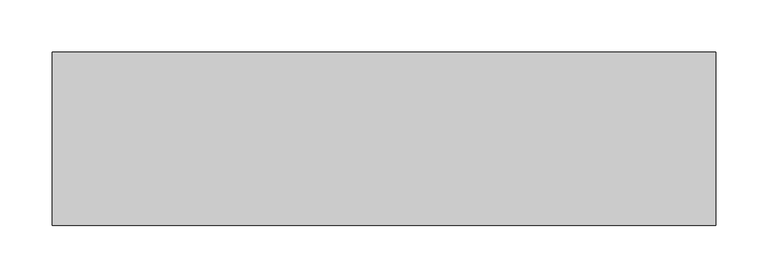
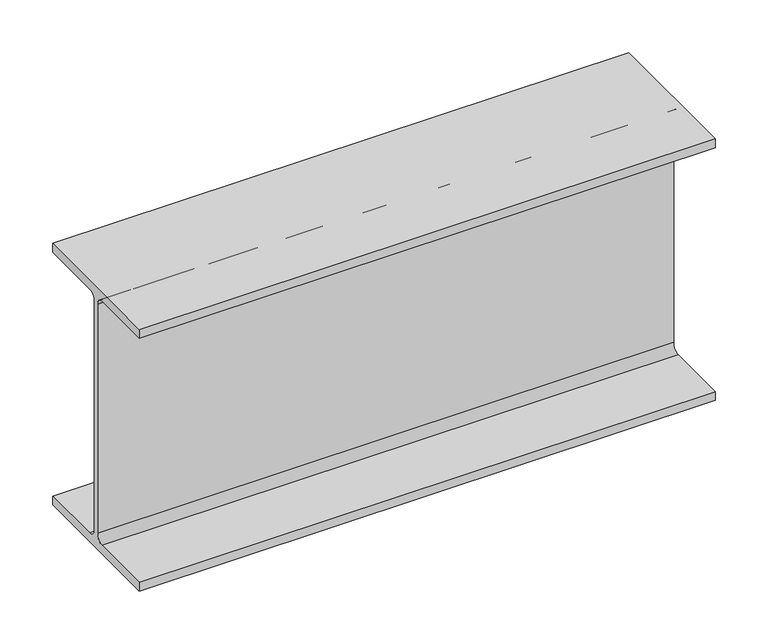
"""IFC4 building model written with IfcOpenShell, lengths in millimetres: beam geometry, Old_Steel Beam_H-KSD3502 : H_SB_ASB_H-300×150x6.5x9."""

from ifc_helpers import new_model, si_unit, point, frame, frame_2d, origin, place, context, project, spatial, polyline, circle_curve, trimmed, segment, composite_curve, outline, extrude, source, transform, mapped, element, save


def beam_aa7ca716(model_context):
    return source(origin(), model_context, "Body", "SweptSolid", [
        extrude(outline(composite_curve([segment(polyline([(-82.5, -141.5), (-11.9, -141.5)]), True, "CONTINUOUS"), segment(trimmed(circle_curve(frame_2d((-11.9, -132.6)), 8.9), [point((-11.9, -141.5))], [point((-3.0, -132.6))], True, "CARTESIAN"), True, "CONTINUOUS"), segment(polyline([(-3.0, -132.6), (-3.0, 132.6)]), True, "CONTINUOUS"), segment(trimmed(circle_curve(frame_2d((-11.9, 132.6)), 8.9), [point((-3.0, 132.6))], [point((-11.9, 141.5))], True, "CARTESIAN"), True, "CONTINUOUS"), segment(polyline([(-11.9, 141.5), (-82.5, 141.5), (-82.5, 151.7), (82.5, 151.7), (82.5, 141.5), (11.9, 141.5)]), True, "CONTINUOUS"), segment(trimmed(circle_curve(frame_2d((11.9, 132.6)), 8.9), [point((11.9, 141.5))], [point((3.0, 132.6))], True, "CARTESIAN"), True, "CONTINUOUS"), segment(polyline([(3.0, 132.6), (3.0, -132.6)]), True, "CONTINUOUS"), segment(trimmed(circle_curve(frame_2d((11.9, -132.6)), 8.9), [point((3.0, -132.6))], [point((11.9, -141.5))], True, "CARTESIAN"), True, "CONTINUOUS"), segment(polyline([(11.9, -141.5), (82.5, -141.5), (82.5, -151.7), (-82.5, -151.7), (-82.5, -141.5)]), True, "CONTINUOUS")], self_intersect=False)), frame((-282.3, 0.0, 0.0), z_axis=(1.0, 0.0, 0.0), x_axis=(0.0, 1.0, 0.0)), (0.0, 0.0, 1.0), 632.1),
    ])


if __name__ == "__main__":
    model = new_model("IFC4")
    model_context = context("Model", 3, world=origin())
    ifc_project = project(units=[si_unit("LENGTHUNIT", "METRE", prefix="MILLI")], contexts=[model_context])
    site = spatial("IfcSite", under=ifc_project)
    building = spatial("IfcBuilding", under=site)
    placement = place(None, origin())
    beam_shape = beam_aa7ca716(model_context)
    element("IfcBeam", 1, ObjectType="Old_Steel Beam_H-KSD3502 : H_SB_ASB_H-300×150x6.5x9", at=placement, inside=building, context=model_context, shape_type="MappedRepresentation", body=[
        mapped(beam_shape, transform((0.0, 0.0, 0.0), x_axis=(1.0, 0.0, 0.0), y_axis=(0.0, 1.0, 0.0), z_axis=(0.0, 0.0, 1.0))),
    ])
    save(model, "model.ifc")

# Revit data of these elements
# Type "Old_Steel Beam_H-KSD3502 : H_SB_ASB_H-300×150x6.5x9"
#   Width = 15.0 cm
#   Web Thickness = 0.65 cm
#   Web Fillet = 1.3 cm
#   Warping Constant = 107174.0 cm⁶
#   Torsional Moment of Inertia = 9.9539 cm⁴
#   Torsional Modulus = 1.0 cm³
#   Section Area = 46.78 cm²
#   Plastic Modulus weak axis = 105.0 cm³
#   Plastic Modulus strong axis = 542.0 cm³
#   Perimeter = 1.17 m²/m
#   Nominal Weight = 36.70 kgf/m
#   Moment of Inertia weak axis = 508.00 cm⁴
#   Moment of Inertia strong axis = 7210.00 cm⁴
#   Height = 30.0 cm
#   Flange Thickness = 0.9 cm
#   Elastic Modulus weak axis = 67.7 cm³
#   Elastic Modulus strong axis = 481.0 cm³
#   Centroid Vertical = 15.0 cm
#   Centroid Horizontal = 7.5 cm
#   Length [instance default] = 1.5240 m
#   Structural Material [instance default] = Steel, 45-345
#   Assembly Code = ""
# Element 1 (IfcBeam, "Old_Steel Beam_H-KSD3502 : H_SB_ASB_H-300×150x6.5x9")
#   Structural Material = none
# Materials
#   "Steel, 45-345": class "Metal", colour RGB 189 187 185, transparency 0, Description = "Steel 345 MPa", Cost = 0
